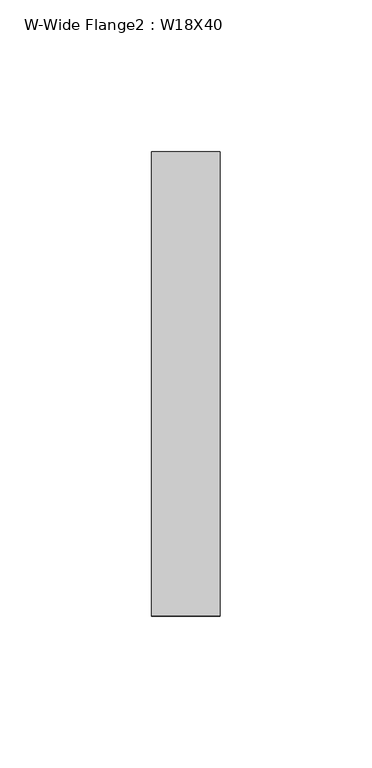
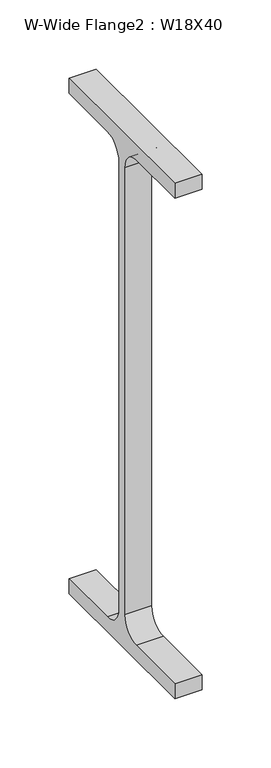
"""IFC4 building model written with IfcOpenShell, lengths in millimetres: beam geometry, W-Wide Flange2 : W18X40."""

from ifc_helpers import new_model, si_unit, point, frame, frame_2d, origin, place, context, project, spatial, polyline, circle_curve, trimmed, segment, composite_curve, outline, extrude, source, transform, mapped, element, save


def w_wide_flange2_w18x40_cd45667b(model_context):
    return source(origin(), model_context, "Body", "SweptSolid", [
        extrude(outline(composite_curve([segment(polyline([(-76.454, -213.995), (-20.828, -213.995)]), True, "CONTINUOUS"), segment(trimmed(circle_curve(frame_2d((-20.828, -197.1675)), 16.8275), [point((-20.828, -213.995))], [point((-4.0005, -197.1675))], True, "CARTESIAN"), True, "CONTINUOUS"), segment(polyline([(-4.0005, -197.1675), (-4.0005, 197.1675)]), True, "CONTINUOUS"), segment(trimmed(circle_curve(frame_2d((-20.828, 197.1675)), 16.8275), [point((-4.0005, 197.1675))], [point((-20.828, 213.995))], True, "CARTESIAN"), True, "CONTINUOUS"), segment(polyline([(-20.828, 213.995), (-76.454, 213.995), (-76.454, 227.33), (76.454, 227.33), (76.454, 213.995), (20.828, 213.995)]), True, "CONTINUOUS"), segment(trimmed(circle_curve(frame_2d((20.828, 197.1675)), 16.8275), [point((20.828, 213.995))], [point((4.0005, 197.1675))], True, "CARTESIAN"), True, "CONTINUOUS"), segment(polyline([(4.0005, 197.1675), (4.0005, -197.1675)]), True, "CONTINUOUS"), segment(trimmed(circle_curve(frame_2d((20.828, -197.1675)), 16.8275), [point((4.0005, -197.1675))], [point((20.828, -213.995))], True, "CARTESIAN"), True, "CONTINUOUS"), segment(polyline([(20.828, -213.995), (76.454, -213.995), (76.454, -227.33), (-76.454, -227.33), (-76.454, -213.995)]), True, "CONTINUOUS")], self_intersect=False)), frame((19.84375, 0.0, 0.0), z_axis=(1.0, 0.0, 0.0), x_axis=(0.0, 1.0, 0.0)), (0.0, 0.0, 1.0), 22.621875),
    ])


if __name__ == "__main__":
    model = new_model("IFC4")
    model_context = context("Model", 3, world=origin())
    ifc_project = project(units=[si_unit("LENGTHUNIT", "METRE", prefix="MILLI")], contexts=[model_context])
    site = spatial("IfcSite", under=ifc_project)
    building = spatial("IfcBuilding", under=site)
    placement = place(None, origin())
    w_wide_flange2_w18x40_shape = w_wide_flange2_w18x40_cd45667b(model_context)
    element("IfcBeam", 1, ObjectType="W-Wide Flange2 : W18X40", at=placement, inside=building, context=model_context, shape_type="MappedRepresentation", body=[
        mapped(w_wide_flange2_w18x40_shape, transform((0.0, 0.0, 0.0), x_axis=(1.0, 0.0, 0.0), y_axis=(0.0, 1.0, 0.0), z_axis=(0.0, 0.0, 1.0))),
    ])
    save(model, "model.ifc")

# Revit data of these elements
# Type "W-Wide Flange2 : W18X40"
#   Assembly Code = "B10"
#   W = 40
#   Length [instance default] = 5' - 0"
#   bf = 0' - 6.02"
#   d = 1' - 5.9"
#   k = 0' - 1 3/16"
#   k2 = 0' - 0.6625"
#   tf = 0' - 0.525"
#   tw = 0' - 0.315"
#   A = 0.0819444 SF
#   Structural Material [instance default] = Steel ASTM A992
# Element 1 (IfcBeam, "W-Wide Flange2 : W18X40")
#   Materials on its faces: "Steel ASTM A992"
# Materials
#   "Steel ASTM A992": class "Metal", colour RGB 199 199 199, transparency 0, Description = "Structural steel 50ksi", Cost = 0
